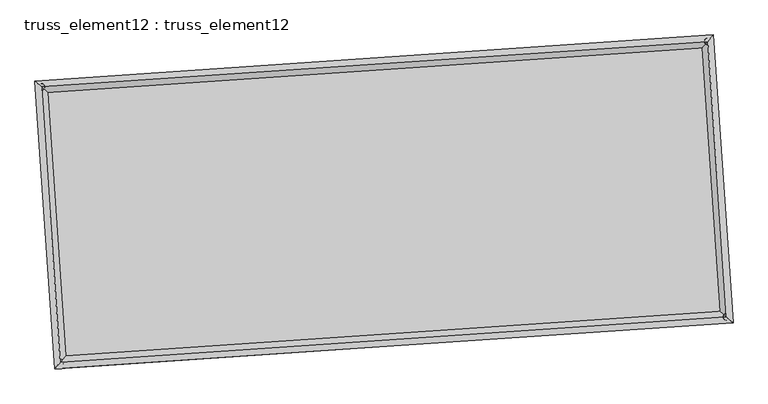
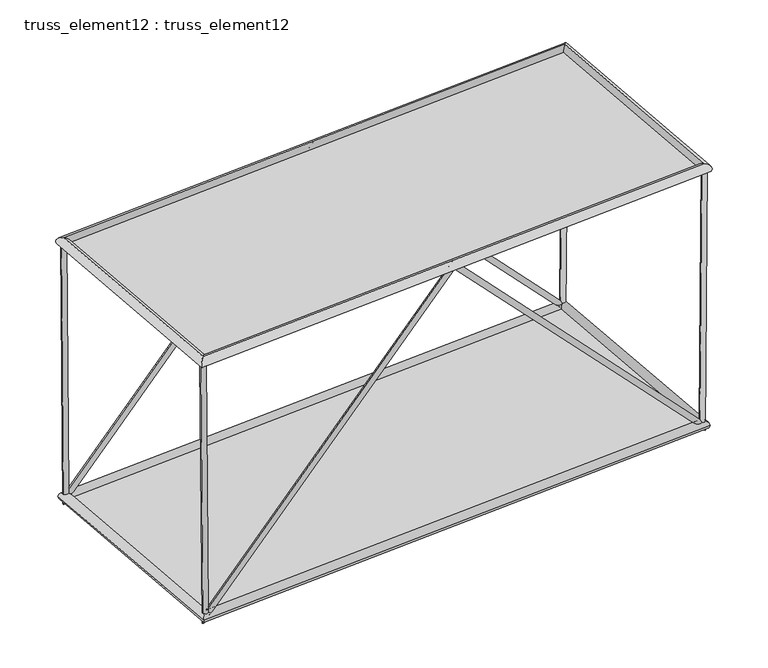
"""IFC4 building model written with IfcOpenShell, lengths in millimetres: plate geometry, truss_element12 : truss_element12."""

from ifc_helpers import new_model, si_unit, frame, origin, origin_with_axes, place, context, project, spatial, polyline, circle_curve, ellipse_curve, outline, extrude, source, transform, mapped, element, save
from ifc_brep_helpers import plane_surface, cylinder_surface, advanced_brep


def truss_element12_truss_element12_5101f613(model_context):
    return source(origin(), model_context, "Body", "SolidModel", [
        advanced_brep(
        [(-3705.894998, 2273.4315212, 5000.2410891), (-3804.9950081, 2260.0704963, 4999.4219397), (-3665.948709, 2276.1553068, 123.1446773), (-3763.0381738, 2262.9313733, -123.1446773), (1064.0644666, 2598.6769247, 5071.9513402), (1064.5075166, 2592.1033628, 4927.7060054), (5793.4043279, 2921.152632, 123.1398302), (5891.3566491, 2921.2278565, -123.1398302), (5834.0188355, 2923.9219809, 5000.2422562), (5934.015137, 2924.1365767, 4999.4094062)],
        [
            (0, 1, circle_curve(frame((-3755.4450031, 2266.7510087, 4999.8315144), z_axis=(-0.008190312331475595, -0.0005584662635913435, 0.9999663028819249), x_axis=(-0.13361032095679876, 0.991033798411517, -0.0005408695425981045)), 50.0)),
            (1, 0, circle_curve(frame((-3755.4450031, 2266.7510087, 4999.8315144), z_axis=(-0.008190312331475595, -0.0005584662635913435, 0.9999663028819249), x_axis=(-0.13361032095679876, 0.991033798411517, -0.0005408695425981045)), 50.0)),
            (0, 2),
            (2, 3, ellipse_curve(frame((-3714.4934414, 2269.54334, 0.0), z_axis=(-0.9272983622915066, -0.06322895033357454, 0.36894423309113283), x_axis=(0.3680895354326023, 0.025098626181828784, 0.9294515333619047)), 132.780268, 50.0)),
            (3, 1),
            (3, 2, ellipse_curve(frame((-3714.4934414, 2269.54334, 0.0), z_axis=(-0.9272983622915066, -0.06322895033357454, 0.36894423309113283), x_axis=(0.3680895354326023, 0.025098626181828784, 0.9294515333619047)), 132.780268, 50.0)),
            (2, 4),
            (4, 5, ellipse_curve(frame((1064.2859916, 2595.3901437, 4999.8286728), z_axis=(-0.9976833954354813, -0.0680282381851024, 3.580167706509558e-05), x_axis=(-3.5718738759339096e-05, -2.4355250164583095e-06, -0.9999999993591201)), 72.2797139, 50.0)),
            (5, 3),
            (5, 4, ellipse_curve(frame((1064.2859916, 2595.3901437, 4999.8286728), z_axis=(-0.9976833954354813, -0.0680282381851024, 3.580167706509558e-05), x_axis=(-3.5718738759339096e-05, -2.4355250164583095e-06, -0.9999999993591201)), 72.2797139, 50.0)),
            (4, 6),
            (6, 7, ellipse_curve(frame((5842.3804885, 2921.1902443, 0.0), z_axis=(-0.9273368066437186, -0.06323157170781109, -0.3688471436560002), x_axis=(-0.3679926709152363, -0.025092021358605998, 0.9294900669812507)), 132.7695372, 50.0)),
            (7, 5),
            (7, 6, ellipse_curve(frame((5842.3804885, 2921.1902443, 0.0), z_axis=(-0.9273368066437186, -0.06323157170781109, -0.3688471436560002), x_axis=(-0.3679926709152363, -0.025092021358605998, 0.9294900669812507)), 132.7695372, 50.0)),
            (8, 9, circle_curve(frame((5884.0169863, 2924.0292788, 4999.8258312), z_axis=(0.008327299552922671, 0.000567806901484687, 0.9999651662320436), x_axis=(-0.0021506121952810596, 0.9999975362268277, -0.0005499158662066811)), 50.0)),
            (9, 8, circle_curve(frame((5884.0169863, 2924.0292788, 4999.8258312), z_axis=(0.008327299552922671, 0.000567806901484687, 0.9999651662320436), x_axis=(-0.0021506121952810596, 0.9999975362268277, -0.0005499158662066811)), 50.0)),
            (6, 8),
            (9, 7),
        ],
        [
            plane_surface(frame((-3755.4450031, 2316.7510009, 4999.8594387), z_axis=(-0.00819031233147702, -0.0005584662635926697, 0.9999663028819249), x_axis=(0.9999664588294515, -4.574166548643177e-06, 0.008190311054175226))),
            cylinder_surface(frame((-3755.4450031, 2266.7510087, 4999.8315144), z_axis=(-0.008190312331475595, -0.0005584662635913435, 0.9999663028819249), x_axis=(-0.13361032095679876, 0.991033798411517, -0.0005408695425981045)), 50.0),
            cylinder_surface(frame((-3714.4934414, 2269.54334, 0.0), z_axis=(-0.6901802934417616, -0.04706077058887605, -0.7221055645930347), x_axis=(-0.02041490918353662, 0.9987521632442915, -0.045577932136905364)), 50.0),
            cylinder_surface(frame((1064.2859916, 2595.3901437, 4999.8286728), z_axis=(-0.6901287062724664, -0.04705725305590286, 0.7221550967164356), x_axis=(-0.11534920510497344, 0.9922789544844527, -0.04557452543792596)), 50.0),
            plane_surface(frame((5884.0169863, 2874.0292868, 4999.8542225), z_axis=(0.008327299552923013, 0.0005678069014865712, 0.9999651662320436), x_axis=(0.9999653274399848, -4.728462105418888e-06, -0.008327298210449648))),
            cylinder_surface(frame((5842.3804885, 2921.1902443, 0.0), z_axis=(-0.008327299552922671, -0.000567806901484687, -0.9999651662320436), x_axis=(-0.0021506121952810596, 0.9999975362268277, -0.0005499158662066811)), 50.0),
        ],
        [
            (0, [[1, 2]]),
            (1, [[-1, 3, 4, 5]]),
            (1, [[-2, -5, 6, -3]]),
            (2, [[-4, 7, 8, 9]]),
            (2, [[-6, -9, 10, -7]]),
            (3, [[-8, 11, 12, 13]]),
            (3, [[-10, -13, 14, -11]]),
            (4, [[15, 16]]),
            (5, [[-12, 17, -16, 18]]),
            (5, [[-14, -18, -15, -17]]),
        ],
    ),
        advanced_brep(
        [(-3433.7820451, -1717.3020631, 5000.2410891), (-3532.8820552, -1730.663088, 4999.4219397), (-3393.8357561, -1714.5782775, 123.1446773), (-3490.9252209, -1727.802211, -123.1446773), (1336.1774195, -1392.0566596, 5071.9513402), (1336.6204695, -1398.6302215, 4927.7060054), (6065.5172808, -1069.5809523, 123.1398302), (6163.469602, -1069.5057278, -123.1398302), (6106.1317884, -1066.8116034, 5000.2422562), (6206.1280899, -1066.5970076, 4999.4094062)],
        [
            (0, 1, circle_curve(frame((-3483.3320502, -1723.9825756, 4999.8315144), z_axis=(-0.008190312331475599, -0.0005584662635913498, 0.9999663028819248), x_axis=(-0.1336103209567986, 0.9910337984115171, -0.0005408695425980977)), 50.0)),
            (1, 0, circle_curve(frame((-3483.3320502, -1723.9825756, 4999.8315144), z_axis=(-0.008190312331475599, -0.0005584662635913498, 0.9999663028819248), x_axis=(-0.1336103209567986, 0.9910337984115171, -0.0005408695425980977)), 50.0)),
            (0, 2),
            (2, 3, ellipse_curve(frame((-3442.3804885, -1721.1902443, 0.0), z_axis=(-0.9272983622915065, -0.06322895033357445, 0.3689442330911329), x_axis=(0.36808953543260237, 0.025098626181828752, 0.9294515333619047)), 132.780268, 50.0)),
            (3, 1),
            (3, 2, ellipse_curve(frame((-3442.3804885, -1721.1902443, 0.0), z_axis=(-0.9272983622915065, -0.06322895033357445, 0.3689442330911329), x_axis=(0.36808953543260237, 0.025098626181828752, 0.9294515333619047)), 132.780268, 50.0)),
            (2, 4),
            (4, 5, ellipse_curve(frame((1336.3989445, -1395.3434406, 4999.8286728), z_axis=(-0.9976833954354813, -0.06802823818510242, 3.580167706565731e-05), x_axis=(-3.571873875995407e-05, -2.435525016391047e-06, -0.9999999993591201)), 72.2797139, 50.0)),
            (5, 3),
            (5, 4, ellipse_curve(frame((1336.3989445, -1395.3434406, 4999.8286728), z_axis=(-0.9976833954354813, -0.06802823818510242, 3.580167706565731e-05), x_axis=(-3.571873875995407e-05, -2.435525016391047e-06, -0.9999999993591201)), 72.2797139, 50.0)),
            (4, 6),
            (6, 7, ellipse_curve(frame((6114.4934414, -1069.54334, 0.0), z_axis=(-0.927336806643719, -0.06323157170781124, -0.36884714365599963), x_axis=(-0.36799267091523563, -0.025092021358605995, 0.9294900669812509)), 132.7695372, 50.0)),
            (7, 5),
            (7, 6, ellipse_curve(frame((6114.4934414, -1069.54334, 0.0), z_axis=(-0.927336806643719, -0.06323157170781124, -0.36884714365599963), x_axis=(-0.36799267091523563, -0.025092021358605995, 0.9294900669812509)), 132.7695372, 50.0)),
            (8, 9, circle_curve(frame((6156.1299392, -1066.7043055, 4999.8258312), z_axis=(0.008327299552923056, 0.0005678069014847247, 0.9999651662320436), x_axis=(-0.00215061219528133, 0.9999975362268277, -0.0005499158662067157)), 50.0)),
            (9, 8, circle_curve(frame((6156.1299392, -1066.7043055, 4999.8258312), z_axis=(0.008327299552923056, 0.0005678069014847247, 0.9999651662320436), x_axis=(-0.00215061219528133, 0.9999975362268277, -0.0005499158662067157)), 50.0)),
            (6, 8),
            (9, 7),
        ],
        [
            plane_surface(frame((-3483.3320502, -1673.9825834, 4999.8594387), z_axis=(-0.00819031233147702, -0.0005584662635926697, 0.9999663028819249), x_axis=(0.9999664588294515, -4.574166548643177e-06, 0.008190311054175226))),
            cylinder_surface(frame((-3483.3320502, -1723.9825756, 4999.8315144), z_axis=(-0.0081903123314756, -0.0005584662635913499, 0.999966302881925), x_axis=(-0.1336103209567986, 0.9910337984115171, -0.0005408695425980977)), 50.0),
            cylinder_surface(frame((-3442.3804885, -1721.1902443, 0.0), z_axis=(-0.6901802934417619, -0.04706077058887601, -0.7221055645930343), x_axis=(-0.020414909183536677, 0.9987521632442914, -0.045577932136905266)), 50.0),
            cylinder_surface(frame((1336.3989445, -1395.3434406, 4999.8286728), z_axis=(-0.6901287062724661, -0.04705725305590294, 0.7221550967164362), x_axis=(-0.11534920510497348, 0.9922789544844528, -0.045574525437925825)), 50.0),
            plane_surface(frame((6156.1299392, -1116.7042975, 4999.8542225), z_axis=(0.008327299552923011, 0.0005678069014865703, 0.9999651662320436), x_axis=(0.9999653274399848, -4.728462104974799e-06, -0.008327298210449648))),
            cylinder_surface(frame((6114.4934414, -1069.54334, 0.0), z_axis=(-0.008327299552923056, -0.0005678069014847247, -0.9999651662320436), x_axis=(-0.00215061219528133, 0.9999975362268277, -0.0005499158662067157)), 50.0),
        ],
        [
            (0, [[1, 2]]),
            (1, [[-1, 3, 4, 5]]),
            (1, [[-2, -5, 6, -3]]),
            (2, [[-4, 7, 8, 9]]),
            (2, [[-6, -9, 10, -7]]),
            (3, [[-8, 11, 12, 13]]),
            (3, [[-10, -13, 14, -11]]),
            (4, [[15, 16]]),
            (5, [[-12, 17, -16, 18]]),
            (5, [[-14, -18, -15, -17]]),
        ],
    ),
        advanced_brep(
        [(-3483.3335482, -1723.9842359, 4909.8315144), (-3483.3305521, -1723.9809152, 5089.8315144), (-3755.4432935, 2266.7495671, 5089.8315144), (-3755.4467126, 2266.7524504, 4909.8315144), (5884.0155938, 2924.0276256, 5089.8258311), (5884.0183787, 2924.0309319, 4909.8258312), (6156.1283353, -1066.7028567, 5089.8258311), (6156.1315431, -1066.7057544, 4909.8258312)],
        [
            (0, 1, ellipse_curve(frame((-3483.3320502, -1723.9825756, 4999.8315144), z_axis=(-0.7535719234053329, 0.6573654662780927, 4.1593136159823963e-07), x_axis=(-0.6573654662779623, -0.7535719234054465, 4.159313615983052e-07)), 127.2792206, 90.0)),
            (1, 2),
            (2, 3, ellipse_curve(frame((-3755.4450031, 2266.7510087, 4999.8315144), z_axis=(-0.6573654662779623, -0.7535719234054467, 4.1593136159836637e-07), x_axis=(0.753571923405333, -0.6573654662780924, -4.1593136159830093e-07)), 127.2792206, 90.0)),
            (3, 0),
            (1, 0, ellipse_curve(frame((-3483.3320502, -1723.9825756, 4999.8315144), z_axis=(-0.7535719234053329, 0.6573654662780927, 4.1593136159823963e-07), x_axis=(-0.6573654662779623, -0.7535719234054465, 4.159313615983052e-07)), 127.2792206, 90.0)),
            (3, 2, ellipse_curve(frame((-3755.4450031, 2266.7510087, 4999.8315144), z_axis=(-0.6573654662779623, -0.7535719234054467, 4.1593136159836637e-07), x_axis=(0.753571923405333, -0.6573654662780924, -4.1593136159830093e-07)), 127.2792206, 90.0)),
            (2, 4),
            (4, 5, ellipse_curve(frame((5884.0169863, 2924.0292788, 4999.8258312), z_axis=(-0.7535719234053329, 0.6573654662780928, 4.159313615983615e-07), x_axis=(-0.6573654662779622, -0.7535719234054467, 4.1593136159830565e-07)), 127.2792206, 90.0)),
            (5, 3),
            (5, 4, ellipse_curve(frame((5884.0169863, 2924.0292788, 4999.8258312), z_axis=(-0.7535719234053329, 0.6573654662780928, 4.159313615983615e-07), x_axis=(-0.6573654662779622, -0.7535719234054467, 4.1593136159830565e-07)), 127.2792206, 90.0)),
            (4, 6),
            (6, 7, ellipse_curve(frame((6156.1299392, -1066.7043055, 4999.8258312), z_axis=(0.6573654662779624, 0.7535719234054465, -4.159313615982445e-07), x_axis=(-0.7535719234053329, 0.6573654662780926, 4.1593136159830035e-07)), 127.2792206, 90.0)),
            (7, 5),
            (7, 6, ellipse_curve(frame((6156.1299392, -1066.7043055, 4999.8258312), z_axis=(0.6573654662779624, 0.7535719234054465, -4.159313615982445e-07), x_axis=(-0.7535719234053329, 0.6573654662780926, 4.1593136159830035e-07)), 127.2792206, 90.0)),
            (6, 1),
            (0, 7),
        ],
        [
            cylinder_surface(frame((-3483.3320502, -1723.9825756, 4999.8315144), z_axis=(0.06802823822869797, -0.9976833960748769, 0.0), x_axis=(-0.9976833959157304, -0.06802823821784637, 1.7861467479703172e-05)), 90.0),
            cylinder_surface(frame((-3755.4450031, 2266.7510087, 4999.8315144), z_axis=(-0.9976833960747045, -0.06802823822868356, 5.882157725886714e-07), x_axis=(-0.06802823820840984, 0.9976833959267312, 1.7273251707202287e-05)), 90.0),
            cylinder_surface(frame((5884.0169863, 2924.0292788, 4999.8258312), z_axis=(-0.06802823822869779, 0.997683396074877, 0.0), x_axis=(0.9976833959360042, 0.06802823821922858, 1.6685035934701416e-05)), 90.0),
            cylinder_surface(frame((6156.1299392, -1066.7043055, 4999.8258312), z_axis=(0.9976833960747044, 0.06802823822868338, -5.882157725885847e-07), x_axis=(0.06802823822868338, -0.9976833959253488, 1.7273251707202294e-05)), 90.0),
        ],
        [
            (0, [[1, 2, 3, 4]]),
            (0, [[5, -4, 6, -2]]),
            (1, [[-3, 7, 8, 9]]),
            (1, [[-6, -9, 10, -7]]),
            (2, [[-8, 11, 12, 13]]),
            (2, [[-10, -13, 14, -11]]),
            (3, [[-12, 15, -1, 16]]),
            (3, [[-14, -16, -5, -15]]),
        ],
    ),
        advanced_brep(
        [(-3358.7115243, -1625.2761972, 0.0), (-3526.0494527, -1817.1042913, 0.0), (-3810.4074885, 2353.2123043, 0.0), (-3618.5793943, 2185.8743758, 0.0), (5926.0494527, 3017.1042913, 0.0), (5758.7115243, 2825.2761972, 0.0), (6210.4074885, -1153.2123043, 0.0), (6018.5793943, -985.8743758, 0.0)],
        [
            (0, 1, ellipse_curve(frame((-3442.3804885, -1721.1902443, 0.0), z_axis=(-0.7535719234054581, 0.6573654662780807, 0.0), x_axis=(-0.6573654662780807, -0.753571923405458, 0.0)), 127.2792206, 90.0)),
            (1, 2),
            (2, 3, ellipse_curve(frame((-3714.4934414, 2269.54334, 0.0), z_axis=(-0.6573654662780808, -0.7535719234054581, 0.0), x_axis=(0.7535719234054581, -0.6573654662780807, 0.0)), 127.2792206, 90.0)),
            (3, 0),
            (1, 0, ellipse_curve(frame((-3442.3804885, -1721.1902443, 0.0), z_axis=(-0.7535719234054581, 0.6573654662780807, 0.0), x_axis=(-0.6573654662780807, -0.753571923405458, 0.0)), 127.2792206, 90.0)),
            (3, 2, ellipse_curve(frame((-3714.4934414, 2269.54334, 0.0), z_axis=(-0.6573654662780808, -0.7535719234054581, 0.0), x_axis=(0.7535719234054581, -0.6573654662780807, 0.0)), 127.2792206, 90.0)),
            (2, 4),
            (4, 5, ellipse_curve(frame((5842.3804885, 2921.1902443, 0.0), z_axis=(-0.7535719234054581, 0.6573654662780807, 0.0), x_axis=(-0.6573654662780808, -0.7535719234054581, 0.0)), 127.2792206, 90.0)),
            (5, 3),
            (5, 4, ellipse_curve(frame((5842.3804885, 2921.1902443, 0.0), z_axis=(-0.7535719234054581, 0.6573654662780807, 0.0), x_axis=(-0.6573654662780808, -0.7535719234054581, 0.0)), 127.2792206, 90.0)),
            (4, 6),
            (6, 7, ellipse_curve(frame((6114.4934414, -1069.54334, 0.0), z_axis=(0.6573654662780808, 0.7535719234054581, 0.0), x_axis=(-0.7535719234054581, 0.6573654662780807, 0.0)), 127.2792206, 90.0)),
            (7, 5),
            (7, 6, ellipse_curve(frame((6114.4934414, -1069.54334, 0.0), z_axis=(0.6573654662780808, 0.7535719234054581, 0.0), x_axis=(-0.7535719234054581, 0.6573654662780807, 0.0)), 127.2792206, 90.0)),
            (6, 1),
            (0, 7),
        ],
        [
            cylinder_surface(frame((-3442.3804885, -1721.1902443, 0.0), z_axis=(0.06802823822870269, -0.9976833960748764, 0.0), x_axis=(-0.9976833960748764, -0.06802823822870269, 0.0)), 90.0),
            cylinder_surface(frame((-3714.4934414, 2269.54334, 0.0), z_axis=(-0.9976833960748767, -0.06802823822870022, 0.0), x_axis=(-0.06802823822870022, 0.9976833960748767, 0.0)), 90.0),
            cylinder_surface(frame((5842.3804885, 2921.1902443, 0.0), z_axis=(-0.06802823822870267, 0.9976833960748764, 0.0), x_axis=(0.9976833960748764, 0.06802823822870267, 0.0)), 90.0),
            cylinder_surface(frame((6114.4934414, -1069.54334, 0.0), z_axis=(0.9976833960748767, 0.0680282382287002, 0.0), x_axis=(0.0680282382287002, -0.9976833960748767, 0.0)), 90.0),
        ],
        [
            (0, [[1, 2, 3, 4]]),
            (0, [[5, -4, 6, -2]]),
            (1, [[-3, 7, 8, 9]]),
            (1, [[-6, -9, 10, -7]]),
            (2, [[-8, 11, 12, 13]]),
            (2, [[-10, -13, 14, -11]]),
            (3, [[-12, 15, -1, 16]]),
            (3, [[-14, -16, -5, -15]]),
        ],
    ),
        extrude(outline(polyline([(-3442.3804885, -1721.1902443), (-3714.4934414, 2269.54334), (5842.3804885, 2921.1902443), (6114.4934414, -1069.54334), (-3442.3804885, -1721.1902443)])), origin_with_axes(), (0.0, 0.0, 1.0), 20.0),
        extrude(outline(polyline([(-2000.0, 4830.9223284), (2000.0, 4830.9223284), (2000.0, -4830.9223283), (-2000.0, -4830.9223283), (-2000.0, 4830.9223284)])), frame((1200.3424681, 600.0233516, 4999.8286728), z_axis=(5.868531096210298e-07, 4.001528270753975e-08, 0.9999999999998271), x_axis=(-0.06802823822870295, 0.9976833960748765, 0.0)), (0.0, 0.0, 1.0), 20.0),
    ])


if __name__ == "__main__":
    model = new_model("IFC4")
    model_context = context("Model", 3, world=origin())
    ifc_project = project(units=[si_unit("LENGTHUNIT", "METRE", prefix="MILLI")], contexts=[model_context])
    site = spatial("IfcSite", under=ifc_project)
    building = spatial("IfcBuilding", under=site)
    placement = place(None, origin())
    truss_element12_truss_element12_shape = truss_element12_truss_element12_5101f613(model_context)
    element("IfcPlate", 1, ObjectType="truss_element12 : truss_element12", at=placement, inside=building, context=model_context, shape_type="MappedRepresentation", body=[
        mapped(truss_element12_truss_element12_shape, transform((0.0, 0.0, 0.0), x_axis=(1.0, 0.0, 0.0), y_axis=(0.0, 1.0, 0.0), z_axis=(0.0, 0.0, 1.0))),
    ])
    save(model, "model.ifc")

# Revit data of these elements
# Type "truss_element12 : truss_element12"
#   steellbar1 = 90 mm
#   steelbar2 = 50 mm
#   offset1 = 5000 mm
#   M = Default Roof
# Element 1 (IfcPlate, "truss_element12 : truss_element12")
#   Materials on its faces: "Default Roof"
# Materials
#   "Default Roof": class "Miscellaneous", colour RGB 0 127 0, transparency 0, Comments = "Rendering appearance not upgraded Rendering appearance not upgraded ", Cost = 0
